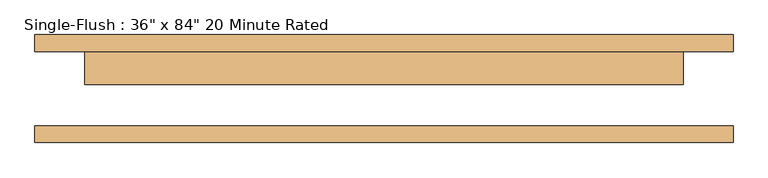
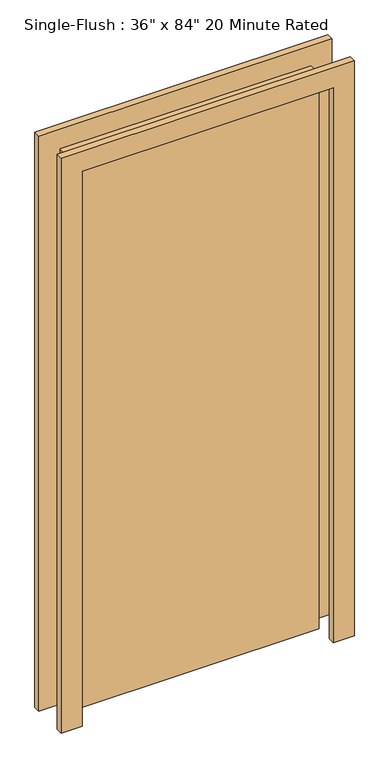
"""IFC4 building model written with IfcOpenShell, lengths in millimetres: door geometry."""

from ifc_helpers import new_model, si_unit, frame, origin, origin_with_axes, place, context, project, spatial, polyline, outline, extrude, source, transform, mapped, element, save


def door_e5f9f3c4(model_context):
    return source(origin(), model_context, "Body", "SweptSolid", [
        extrude(outline(polyline([(2209.8, -533.4), (0.0, -533.4), (0.0, -457.2), (2133.6, -457.2), (2133.6, 457.2), (0.0, 457.2), (0.0, 533.4), (2209.8, 533.4), (2209.8, -533.4)])), frame((0.0, 57.15, 0.0), z_axis=(0.0, 1.0, 0.0), x_axis=(0.0, 0.0, 1.0)), (0.0, 0.0, 1.0), 25.4),
        extrude(outline(polyline([(2209.8, 533.4), (2209.8, -533.4), (0.0, -533.4), (0.0, -457.2), (2133.6, -457.2), (2133.6, 457.2), (0.0, 457.2), (0.0, 533.4), (2209.8, 533.4)])), frame((0.0, -82.55, 0.0), z_axis=(0.0, 1.0, 0.0), x_axis=(0.0, 0.0, 1.0)), (0.0, 0.0, 1.0), 25.4),
        extrude(outline(polyline([(457.2, 6.35), (-457.2, 6.35), (-457.2, 57.15), (457.2, 57.15), (457.2, 6.35)])), origin_with_axes(), (0.0, 0.0, 1.0), 2133.6),
    ])


if __name__ == "__main__":
    model = new_model("IFC4")
    model_context = context("Model", 3, world=origin())
    ifc_project = project(units=[si_unit("LENGTHUNIT", "METRE", prefix="MILLI")], contexts=[model_context])
    site = spatial("IfcSite", under=ifc_project)
    building = spatial("IfcBuilding", under=site)
    placement = place(None, origin())
    door_shape = door_e5f9f3c4(model_context)
    element("IfcDoor", 1, ObjectType="Single-Flush : 36\" x 84\" 20 Minute Rated", at=placement, inside=building, context=model_context, shape_type="MappedRepresentation", body=[
        mapped(door_shape, transform((0.0, 0.0, 0.0), x_axis=(1.0, 0.0, 0.0), y_axis=(0.0, 1.0, 0.0), z_axis=(0.0, 0.0, 1.0))),
    ])
    save(model, "model.ifc")

# Revit data of these elements
# Type "Single-Flush : 36\" x 84\" 20 Minute Rated"
#   Type Mark = "20"
#   Fire Rating = "20 Min."
#   Assembly Code = "C1020"
#   Thickness = 0' - 2"
#   Height = 7' - 0"
#   Trim Projection Ext = 0' - 1"
#   Trim Projection Int = 0' - 1"
#   Trim Width = 0' - 3"
#   Width = 3' - 0"
#   Function = 0
#   Door Material = Door - Panel
#   Frame Material = Door - Frame
#   Wall Closure = (empty or 0)
# Element 1 (IfcDoor, "Single-Flush : 36\" x 84\" 20 Minute Rated")
#   Materials on its faces: "Door - Frame", "Door - Panel"
# Materials
#   "Door - Panel": class "Wood", colour RGB 210 159 95, transparency 0
#   "Door - Frame": class "Miscellaneous", colour RGB 118 70 51, transparency 0
